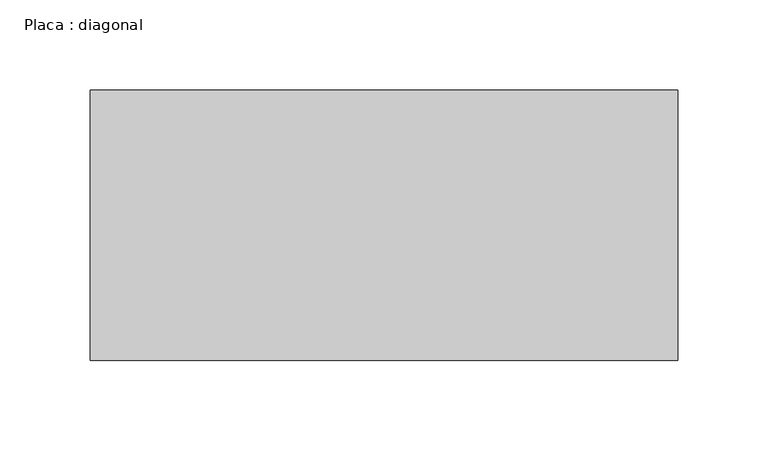
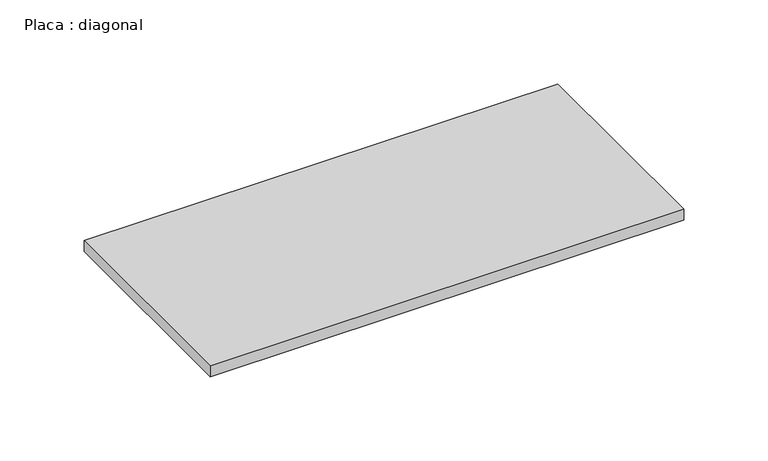
"""IFC4 building model written with IfcOpenShell, lengths in millimetres: beam geometry, Placa : diagonal."""

from ifc_helpers import new_model, si_unit, frame, origin, place, context, project, spatial, polyline, outline, extrude, source, transform, mapped, element, save


def placa_diagonal_67ce8334(model_context):
    return source(origin(), model_context, "Body", "SweptSolid", [
        extrude(outline(polyline([(162.9623469, 75.0), (162.9623469, -75.0), (-162.6761246, -75.0), (-162.6761246, 75.0), (162.9623469, 75.0)])), frame((0.0, 0.0, -4.0), z_axis=(0.0, 0.0, 1.0), x_axis=(1.0, 0.0, 0.0)), (0.0, 0.0, 1.0), 8.0),
    ])


if __name__ == "__main__":
    model = new_model("IFC4")
    model_context = context("Model", 3, world=origin())
    ifc_project = project(units=[si_unit("LENGTHUNIT", "METRE", prefix="MILLI")], contexts=[model_context])
    site = spatial("IfcSite", under=ifc_project)
    building = spatial("IfcBuilding", under=site)
    placement = place(None, origin())
    placa_diagonal_shape = placa_diagonal_67ce8334(model_context)
    element("IfcBeam", 1, ObjectType="Placa : diagonal", at=placement, inside=building, context=model_context, shape_type="MappedRepresentation", body=[
        mapped(placa_diagonal_shape, transform((0.0, 0.0, 0.0), x_axis=(1.0, 0.0, 0.0), y_axis=(0.0, 1.0, 0.0), z_axis=(0.0, 0.0, 1.0))),
    ])
    save(model, "model.ifc")

# Revit data of these elements
# Type "Placa : diagonal"
#   W = 0
#   Length [instance default] = 1.50 m
#   b = 0.15 m
#   d = 0.008 m
#   A = 0 m²
#   Structural Material [instance default] = Aço, 45-345
# Element 1 (IfcBeam, "Placa : diagonal")
#   Materials on its faces: "Aço, 45-345"
# Materials
#   "Aço, 45-345": class "Metal", colour RGB 247 247 247, transparency 0, Description = "Aço 345 MPa", Cost = 0
